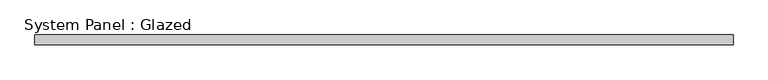
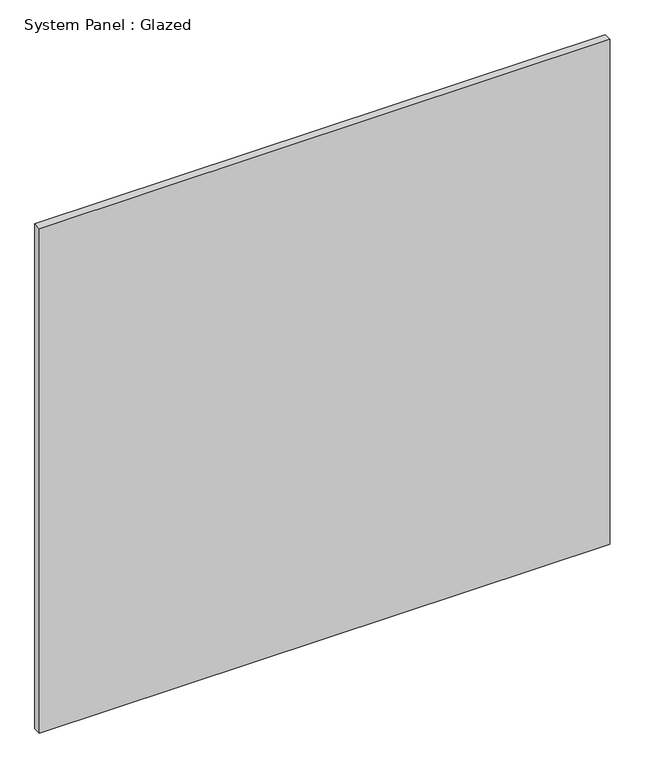
"""IFC4 building model written with IfcOpenShell, lengths in millimetres: plate geometry, System Panel : Glazed."""

import ifcopenshell
import ifcopenshell.guid

model = None  # the IFC model being written
_history = None  # IfcOwnerHistory: only IFC2X3 demands one
_inside = {}  # id of a spatial element -> (the spatial element, [elements in it])
_under = {}  # id of a project, library or spatial element -> (it, [spatial elements below it])
_declared = {}  # id of a project -> (the project, [libraries it declares])
_typed = {}  # id of a type object -> (the type object, [elements of that type])
_made_of = {}  # id of a material, layer set ... -> (it, [elements and type objects made of it])


def new_model(schema):
    """Start an empty IFC model of exactly this schema.

    Asked for "IFC4X3", IfcOpenShell would pick the latest addendum, in which some entities
    have other attributes; the version numbers below select the first issue.
    IFC2X3 requires an IfcOwnerHistory on every rooted entity: one is made here for all.
    """
    global model, _history
    if schema == "IFC4X3":
        model = ifcopenshell.file(schema_version=(4, 3, 0, 0))
    else:
        model = ifcopenshell.file(schema=schema)
    _inside.clear()
    _under.clear()
    _declared.clear()
    _typed.clear()
    _made_of.clear()
    _history = None
    if model.schema == "IFC2X3":
        org = make("IfcOrganization", Name="unknown")
        user = make(
            "IfcPersonAndOrganization",
            ThePerson=make("IfcPerson", FamilyName="unknown"),
            TheOrganization=org,
        )
        app = make(
            "IfcApplication",
            ApplicationDeveloper=org,
            Version="unknown",
            ApplicationFullName="unknown",
            ApplicationIdentifier="unknown",
        )
        _history = make(
            "IfcOwnerHistory",
            OwningUser=user,
            OwningApplication=app,
            ChangeAction="ADDED",
            CreationDate=0,
        )
    return model


def make(cls, **values):
    """One entity of the class cls with the attributes given. An attribute that is None is left unset."""
    return model.create_entity(
        cls, **{name: value for name, value in values.items() if value is not None}
    )


def rooted(cls, **values):
    """An entity with a GlobalId (a new one), such as an element, a storey or a relation."""
    return make(cls, GlobalId=ifcopenshell.guid.new(), OwnerHistory=_history, **values)


def si_unit(unit_type, name, prefix=None):
    """IfcSIUnit, for example si_unit("LENGTHUNIT", "METRE", prefix="MILLI")."""
    return make("IfcSIUnit", UnitType=unit_type, Prefix=prefix, Name=name)


def assignment(units):
    """IfcUnitAssignment: the units of a project."""
    return None if units is None else make("IfcUnitAssignment", Units=units)


def point(xyz):
    """IfcCartesianPoint."""
    return None if xyz is None else make("IfcCartesianPoint", Coordinates=xyz)


def direction(xyz):
    """IfcDirection."""
    return None if xyz is None else make("IfcDirection", DirectionRatios=xyz)


def frame(location, z_axis=None, x_axis=None):
    """IfcAxis2Placement3D, a coordinate frame: its origin and axes. An axis left out is left unset."""
    return make(
        "IfcAxis2Placement3D",
        Location=point(location),
        Axis=direction(z_axis),
        RefDirection=direction(x_axis),
    )


def origin():
    """The frame at (0, 0, 0) with its axes left unset."""
    return frame((0.0, 0.0, 0.0))


def origin_with_axes():
    """The frame at (0, 0, 0) with the z axis (0, 0, 1) and the x axis (1, 0, 0) written out."""
    return frame((0.0, 0.0, 0.0), z_axis=(0.0, 0.0, 1.0), x_axis=(1.0, 0.0, 0.0))


def place(relative_to, where):
    """IfcLocalPlacement: puts the frame where relative to a parent placement (None: the world)."""
    return make(
        "IfcLocalPlacement", PlacementRelTo=relative_to, RelativePlacement=where
    )


def context(
    kind, dimensions, precision=None, world=None, true_north=None, identifier=None
):
    """IfcGeometricRepresentationContext, for example the 3D "Model" context."""
    return make(
        "IfcGeometricRepresentationContext",
        ContextIdentifier=identifier,
        ContextType=kind,
        CoordinateSpaceDimension=dimensions,
        Precision=precision,
        WorldCoordinateSystem=world,
        TrueNorth=true_north,
    )


def project(units=None, contexts=None):
    """IfcProject with its units and contexts."""
    return rooted(
        "IfcProject",
        Name="project",
        RepresentationContexts=contexts,
        UnitsInContext=assignment(units),
    )


def spatial(cls, under=None, at=None, **own):
    """A site, building, storey or space (cls), placed at a placement, below another one or the project."""
    s = rooted(cls, ObjectPlacement=at, **own)
    if under is not None:
        _under.setdefault(under.id(), (under, []))[1].append(s)
    return s


def polyline(points):
    """IfcPolyline through the points."""
    return make("IfcPolyline", Points=[point(p) for p in points])


def outline(outer, holes=None, kind="AREA"):
    """IfcArbitraryClosedProfileDef: a profile drawn as a closed curve; with holes, ...WithVoids."""
    if holes is None:
        return make("IfcArbitraryClosedProfileDef", ProfileType=kind, OuterCurve=outer)
    return make(
        "IfcArbitraryProfileDefWithVoids",
        ProfileType=kind,
        OuterCurve=outer,
        InnerCurves=holes,
    )


def extrude(swept, where, along, depth):
    """IfcExtrudedAreaSolid: the profile swept, set in the frame where, extruded along a direction by depth."""
    return make(
        "IfcExtrudedAreaSolid",
        SweptArea=swept,
        Position=where,
        ExtrudedDirection=direction(along),
        Depth=depth,
    )


def shape(context_of_items, identifier, shape_type, items):
    """IfcShapeRepresentation: the items that make up one representation, for example the "Body"."""
    return make(
        "IfcShapeRepresentation",
        ContextOfItems=context_of_items,
        RepresentationIdentifier=identifier,
        RepresentationType=shape_type,
        Items=items,
    )


def source(mapping_origin, context_of_items, identifier, shape_type, items):
    """IfcRepresentationMap: a shape defined once, which mapped items show again and again."""
    return make(
        "IfcRepresentationMap",
        MappingOrigin=mapping_origin,
        MappedRepresentation=shape(context_of_items, identifier, shape_type, items),
    )


def transform(
    local_origin,
    x_axis=None,
    y_axis=None,
    z_axis=None,
    scale=None,
    scale2=None,
    scale3=None,
    uniform=True,
):
    """IfcCartesianTransformationOperator3D, or its non-uniform kind. x_axis, y_axis, z_axis: its Axis1, 2, 3."""
    if uniform:
        return make(
            "IfcCartesianTransformationOperator3D",
            Axis1=direction(x_axis),
            Axis2=direction(y_axis),
            LocalOrigin=point(local_origin),
            Scale=scale,
            Axis3=direction(z_axis),
        )
    return make(
        "IfcCartesianTransformationOperator3DnonUniform",
        Axis1=direction(x_axis),
        Axis2=direction(y_axis),
        LocalOrigin=point(local_origin),
        Scale=scale,
        Axis3=direction(z_axis),
        Scale2=scale2,
        Scale3=scale3,
    )


def mapped(mapping_source, mapping_target):
    """IfcMappedItem: shows the shape of a source again, moved by a transform."""
    return make(
        "IfcMappedItem", MappingSource=mapping_source, MappingTarget=mapping_target
    )


def made_of(thing, what):
    """Note that an element or type object is made of a material, layer set ...; save() writes the relation."""
    if what is not None:
        _made_of.setdefault(what.id(), (what, []))[1].append(thing)
    return thing


def element(
    cls,
    number,
    at=None,
    inside=None,
    cuts=None,
    type_object=None,
    material=None,
    context=None,
    identifier="Body",
    shape_type=None,
    held_by="IfcProductDefinitionShape",
    body=None,
    shapes=None,
    **own,
):
    """One element of the class cls, such as IfcWall. Its Tag is "e" and its number.

    at: its placement. inside: the storey or other place that contains it. cuts: it is an
    opening in that element (IfcRelVoidsElement). A single representation is given by context,
    identifier, shape_type and body (its items); several are given by shapes. held_by: the class
    of the entity that holds the representations. save() writes the other relations.
    """
    e = rooted(cls, Tag="e%d" % number, ObjectPlacement=at, **own)
    if body is not None:
        shapes = [shape(context, identifier, shape_type, body)]
    if shapes is not None:
        e.Representation = make(held_by, Representations=shapes)
    if inside is not None:
        _inside.setdefault(inside.id(), (inside, []))[1].append(e)
    if cuts is not None:
        rooted(
            "IfcRelVoidsElement", RelatingBuildingElement=cuts, RelatedOpeningElement=e
        )
    if type_object is not None:
        _typed.setdefault(type_object.id(), (type_object, []))[1].append(e)
    return made_of(e, material)


def aggregate(whole, parts):
    """IfcRelAggregates: a whole, such as a stair, and the parts it consists of."""
    return rooted("IfcRelAggregates", RelatingObject=whole, RelatedObjects=parts)


def save(model, path):
    """Write the relations noted so far, then the file.

    IfcRelAggregates (storeys below a building ...), IfcRelContainedInSpatialStructure (elements
    in a storey), IfcRelDefinesByType, IfcRelAssociatesMaterial and IfcRelDeclares: one each for
    every whole, place, type object, material and project.
    """
    for whole, parts in _under.values():
        aggregate(whole, parts)
    for where, things in _inside.values():
        rooted(
            "IfcRelContainedInSpatialStructure",
            RelatedElements=things,
            RelatingStructure=where,
        )
    for kind, things in _typed.values():
        rooted("IfcRelDefinesByType", RelatedObjects=things, RelatingType=kind)
    for what, things in _made_of.values():
        rooted("IfcRelAssociatesMaterial", RelatedObjects=things, RelatingMaterial=what)
    for by, libraries in _declared.values():
        rooted("IfcRelDeclares", RelatingContext=by, RelatedDefinitions=libraries)
    model.write(path)


def system_panel_glazed_78d7b886(model_context):
    return source(origin(), model_context, "Body", "SweptSolid", [
        extrude(outline(polyline([(902.5000002, 24.5), (-902.5000002, 24.5), (-902.5000002, 49.5), (902.5000002, 49.5), (902.5000002, 24.5)])), origin_with_axes(), (0.0, 0.0, 1.0), 1686.2355347),
    ])


if __name__ == "__main__":
    model = new_model("IFC4")
    model_context = context("Model", 3, world=origin())
    ifc_project = project(units=[si_unit("LENGTHUNIT", "METRE", prefix="MILLI")], contexts=[model_context])
    site = spatial("IfcSite", under=ifc_project)
    building = spatial("IfcBuilding", under=site)
    placement = place(None, origin())
    system_panel_glazed_shape = system_panel_glazed_78d7b886(model_context)
    element("IfcPlate", 1, ObjectType="System Panel : Glazed", at=placement, inside=building, context=model_context, shape_type="MappedRepresentation", body=[
        mapped(system_panel_glazed_shape, transform((0.0, 0.0, 0.0), x_axis=(1.0, 0.0, 0.0), y_axis=(0.0, 1.0, 0.0), z_axis=(0.0, 0.0, 1.0))),
    ])
    save(model, "model.ifc")

# Revit data of these elements
# Element 1 (IfcPlate, "System Panel : Glazed")
#   Materials on its faces: "Glass"
# Materials
#   "Glass": class "Glass", colour RGB 218 227 224, transparency 0.85, Description = "Soda Lime Glass", Cost = 0
